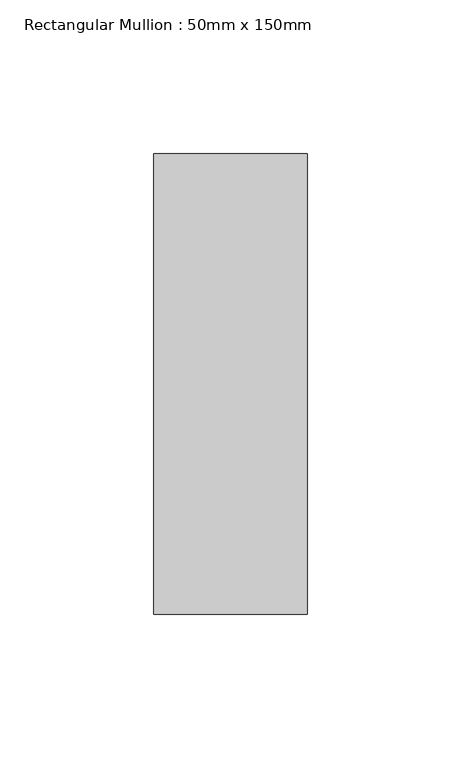
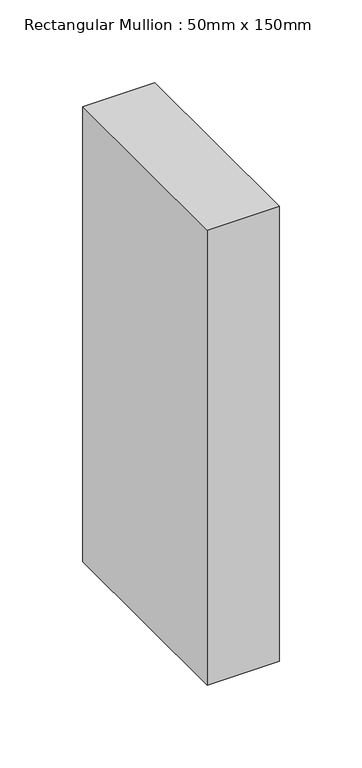
"""IFC4 building model written with IfcOpenShell, lengths in millimetres: member geometry, Rectangular Mullion : 50mm x 150mm."""

from ifc_helpers import new_model, si_unit, frame, origin, place, context, project, spatial, polyline, outline, extrude, source, transform, mapped, element, save


def rectangular_mullion_50mm_x_150mm_374b2159(model_context):
    return source(origin(), model_context, "Body", "SweptSolid", [
        extrude(outline(polyline([(0.0, 75.0), (0.0, -75.0), (-50.0, -75.0), (-50.0, 75.0), (0.0, 75.0)])), frame((0.0, 0.0, -334.8484849), z_axis=(0.0, 0.0, 1.0), x_axis=(1.0, 0.0, 0.0)), (0.0, 0.0, 1.0), 334.8484849),
    ])


if __name__ == "__main__":
    model = new_model("IFC4")
    model_context = context("Model", 3, world=origin())
    ifc_project = project(units=[si_unit("LENGTHUNIT", "METRE", prefix="MILLI")], contexts=[model_context])
    site = spatial("IfcSite", under=ifc_project)
    building = spatial("IfcBuilding", under=site)
    placement = place(None, origin())
    rectangular_mullion_50mm_x_150mm_shape = rectangular_mullion_50mm_x_150mm_374b2159(model_context)
    element("IfcMember", 1, ObjectType="Rectangular Mullion : 50mm x 150mm", at=placement, inside=building, context=model_context, shape_type="MappedRepresentation", body=[
        mapped(rectangular_mullion_50mm_x_150mm_shape, transform((0.0, 0.0, 0.0), x_axis=(1.0, 0.0, 0.0), y_axis=(0.0, 1.0, 0.0), z_axis=(0.0, 0.0, 1.0))),
    ])
    save(model, "model.ifc")

# Revit data of these elements
# Type "Rectangular Mullion : 50mm x 150mm"
#   built-in parameter 1007304 = 0.492126 (stored number, unit not read)
#   built-in parameter 1007301 = 0.082021 (stored number, unit not read)
#   built-in parameter 1007300 = 0.082021 (stored number, unit not read)
# Element 1 (IfcMember, "Rectangular Mullion : 50mm x 150mm")
#   Materials on its faces: "Aluminum"
# Materials
#   "Aluminum": class "Metal", colour RGB 244 244 244, transparency 0, Description = "Aluminum 6061", Cost = 0
